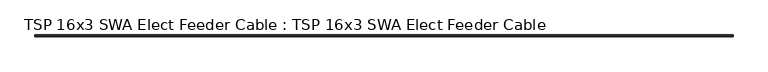
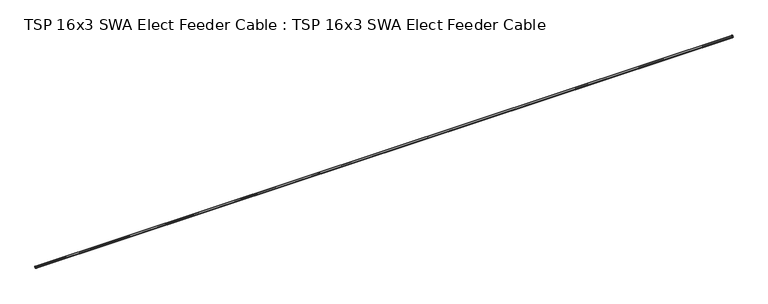
"""IFC4 building model written with IfcOpenShell, lengths in millimetres: proxy geometry, TSP 16x3 SWA Elect Feeder Cable : TSP 16x3 SWA Elect Feeder Cable."""

from ifc_helpers import new_model, si_unit, point, frame, frame_2d, origin, origin_2d, place, context, project, spatial, circle_curve, trimmed, segment, composite_curve, outline, extrude, source, transform, mapped, element, save


def tsp_16x3_swa_elect_feeder_cable_tsp_16x3_swa_elect_feeder_479ea12e(model_context):
    return source(origin(), model_context, "Body", "SweptSolid", [
        extrude(outline(composite_curve([segment(trimmed(circle_curve(origin_2d(), 30.0), [point((-30.0, 0.0))], [point((30.0, 0.0))], False, "CARTESIAN"), True, "CONTINUOUS"), segment(trimmed(circle_curve(origin_2d(), 30.0), [point((30.0, 0.0))], [point((-30.0, 0.0))], False, "CARTESIAN"), True, "CONTINUOUS")], self_intersect=False), holes=[composite_curve([segment(trimmed(circle_curve(origin_2d(), 27.0), [point((-27.0, 0.0))], [point((27.0, 0.0))], True, "CARTESIAN"), True, "CONTINUOUS"), segment(trimmed(circle_curve(origin_2d(), 27.0), [point((27.0, 0.0))], [point((-27.0, 0.0))], True, "CARTESIAN"), True, "CONTINUOUS")], self_intersect=False)]), frame((0.0, 0.0, 0.0), z_axis=(1.0, 0.0, 0.0), x_axis=(0.0, 1.0, 0.0)), (0.0, 0.0, 1.0), 21159.3895389),
        extrude(outline(composite_curve([segment(trimmed(circle_curve(frame_2d((11.691343, 6.75)), 8.0), [point((3.691343, 6.75))], [point((19.691343, 6.75))], False, "CARTESIAN"), True, "CONTINUOUS"), segment(trimmed(circle_curve(frame_2d((11.691343, 6.75)), 8.0), [point((19.691343, 6.75))], [point((3.691343, 6.75))], False, "CARTESIAN"), True, "CONTINUOUS")], self_intersect=False)), frame((0.0, 0.0, 0.0), z_axis=(1.0, 0.0, 0.0), x_axis=(0.0, 1.0, 0.0)), (0.0, 0.0, 1.0), 21159.3895389),
        extrude(outline(composite_curve([segment(trimmed(circle_curve(frame_2d((-11.691343, 6.75)), 8.0), [point((-19.691343, 6.75))], [point((-3.691343, 6.75))], False, "CARTESIAN"), True, "CONTINUOUS"), segment(trimmed(circle_curve(frame_2d((-11.691343, 6.75)), 8.0), [point((-3.691343, 6.75))], [point((-19.691343, 6.75))], False, "CARTESIAN"), True, "CONTINUOUS")], self_intersect=False)), frame((0.0, 0.0, 0.0), z_axis=(1.0, 0.0, 0.0), x_axis=(0.0, 1.0, 0.0)), (0.0, 0.0, 1.0), 21159.3895389),
        extrude(outline(composite_curve([segment(trimmed(circle_curve(frame_2d((0.0, -13.5)), 8.0), [point((-8.0, -13.5))], [point((8.0, -13.5))], False, "CARTESIAN"), True, "CONTINUOUS"), segment(trimmed(circle_curve(frame_2d((0.0, -13.5)), 8.0), [point((8.0, -13.5))], [point((-8.0, -13.5))], False, "CARTESIAN"), True, "CONTINUOUS")], self_intersect=False)), frame((0.0, 0.0, 0.0), z_axis=(1.0, 0.0, 0.0), x_axis=(0.0, 1.0, 0.0)), (0.0, 0.0, 1.0), 21159.3895389),
        extrude(outline(composite_curve([segment(trimmed(circle_curve(origin_2d(), 27.0), [point((27.0, 0.0))], [point((-27.0, 0.0))], False, "CARTESIAN"), True, "CONTINUOUS"), segment(trimmed(circle_curve(origin_2d(), 27.0), [point((-27.0, 0.0))], [point((27.0, 0.0))], False, "CARTESIAN"), True, "CONTINUOUS")], self_intersect=False), holes=[composite_curve([segment(trimmed(circle_curve(frame_2d((-11.691343, 6.75)), 8.0), [point((-3.691343, 6.75))], [point((-19.691343, 6.75))], True, "CARTESIAN"), True, "CONTINUOUS"), segment(trimmed(circle_curve(frame_2d((-11.691343, 6.75)), 8.0), [point((-19.691343, 6.75))], [point((-3.691343, 6.75))], True, "CARTESIAN"), True, "CONTINUOUS")], self_intersect=False), composite_curve([segment(trimmed(circle_curve(frame_2d((11.691343, 6.75)), 8.0), [point((3.691343, 6.75))], [point((19.691343, 6.75))], True, "CARTESIAN"), True, "CONTINUOUS"), segment(trimmed(circle_curve(frame_2d((11.691343, 6.75)), 8.0), [point((19.691343, 6.75))], [point((3.691343, 6.75))], True, "CARTESIAN"), True, "CONTINUOUS")], self_intersect=False), composite_curve([segment(trimmed(circle_curve(frame_2d((0.0, -13.5)), 8.0), [point((-8.0, -13.5))], [point((8.0, -13.5))], True, "CARTESIAN"), True, "CONTINUOUS"), segment(trimmed(circle_curve(frame_2d((0.0, -13.5)), 8.0), [point((8.0, -13.5))], [point((-8.0, -13.5))], True, "CARTESIAN"), True, "CONTINUOUS")], self_intersect=False)]), frame((0.0, 0.0, 0.0), z_axis=(1.0, 0.0, 0.0), x_axis=(0.0, 1.0, 0.0)), (0.0, 0.0, 1.0), 21159.3895389),
    ])


if __name__ == "__main__":
    model = new_model("IFC4")
    model_context = context("Model", 3, world=origin())
    ifc_project = project(units=[si_unit("LENGTHUNIT", "METRE", prefix="MILLI")], contexts=[model_context])
    site = spatial("IfcSite", under=ifc_project)
    building = spatial("IfcBuilding", under=site)
    placement = place(None, origin())
    tsp_16x3_swa_elect_feeder_cable_tsp_16x3_swa_elect_feeder_shape = tsp_16x3_swa_elect_feeder_cable_tsp_16x3_swa_elect_feeder_479ea12e(model_context)
    element("IfcBuildingElementProxy", 1, Name="TSP 16x3 SWA Elect Feeder Cable : TSP 16x3 SWA Elect Feeder Cable", ObjectType="TSP 16x3 SWA Elect Feeder Cable : TSP 16x3 SWA Elect Feeder Cable", at=placement, inside=building, context=model_context, shape_type="MappedRepresentation", body=[
        mapped(tsp_16x3_swa_elect_feeder_cable_tsp_16x3_swa_elect_feeder_shape, transform((0.0, 0.0, 0.0), x_axis=(1.0, 0.0, 0.0), y_axis=(0.0, 1.0, 0.0), z_axis=(0.0, 0.0, 1.0))),
    ])
    save(model, "model.ifc")

# Revit data of these elements
# Type "TSP 16x3 SWA Elect Feeder Cable : TSP 16x3 SWA Elect Feeder Cable"
#   Model = "TSP_ELECSC163"
#   built-in parameter 1001306 [instance default] = 3.93701 (stored number, unit not read)
#   Cable Length [instance default] = 1200 mm
#   Default Elevation = 0
# Element 1 (IfcBuildingElementProxy, "TSP 16x3 SWA Elect Feeder Cable : TSP 16x3 SWA Elect Feeder Cable")
#   built-in parameter 1001306 = 69.4206 (stored number, unit not read)
#   Cable Length = 21159.39 mm
#   Materials on its faces: "Cellulose Fill", "Copper", "Laminate, Red, Matte"
# Materials
#   "Cellulose Fill": class "Generic", colour RGB 0 0 0, transparency 0, Description = "Cellulose loose fill", Cost = 0
#   "Copper": class "Metal", colour RGB 0 0 0, transparency 0, Description = "Copper, matte finish", Cost = 0
#   "Laminate, Red, Matte": class "Plastic", colour RGB 255 0 0, transparency 0, Description = "Plastic Laminate - Red, Matte", Cost = 0
